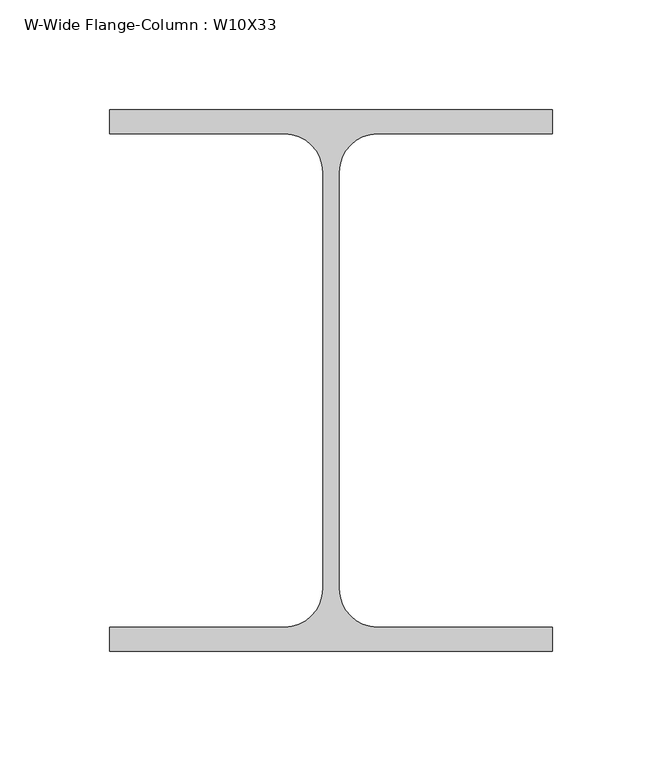
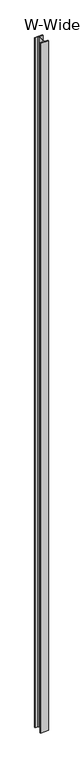
"""IFC4 building model written with IfcOpenShell, lengths in millimetres: column geometry, W-Wide Flange-Column : W10X33."""

from ifc_helpers import new_model, si_unit, point, frame, frame_2d, origin, place, context, project, spatial, polyline, circle_curve, trimmed, segment, composite_curve, outline, extrude, source, transform, mapped, element, save


def w_wide_flange_column_w10x33_d5634f11(model_context):
    return source(origin(), model_context, "Body", "SweptSolid", [
        extrude(outline(composite_curve([segment(polyline([(101.092, 123.571), (101.092, 112.522), (21.209, 112.522)]), True, "CONTINUOUS"), segment(trimmed(circle_curve(frame_2d((21.209, 94.996)), 17.526), [point((21.209, 112.522))], [point((3.683, 94.996))], True, "CARTESIAN"), True, "CONTINUOUS"), segment(polyline([(3.683, 94.996), (3.683, -94.996)]), True, "CONTINUOUS"), segment(trimmed(circle_curve(frame_2d((21.209, -94.996)), 17.526), [point((3.683, -94.996))], [point((21.209, -112.522))], True, "CARTESIAN"), True, "CONTINUOUS"), segment(polyline([(21.209, -112.522), (101.092, -112.522), (101.092, -123.571), (-101.092, -123.571), (-101.092, -112.522), (-21.209, -112.522)]), True, "CONTINUOUS"), segment(trimmed(circle_curve(frame_2d((-21.209, -94.996)), 17.526), [point((-21.209, -112.522))], [point((-3.683, -94.996))], True, "CARTESIAN"), True, "CONTINUOUS"), segment(polyline([(-3.683, -94.996), (-3.683, 94.996)]), True, "CONTINUOUS"), segment(trimmed(circle_curve(frame_2d((-21.209, 94.996)), 17.526), [point((-3.683, 94.996))], [point((-21.209, 112.522))], True, "CARTESIAN"), True, "CONTINUOUS"), segment(polyline([(-21.209, 112.522), (-101.092, 112.522), (-101.092, 123.571), (101.092, 123.571)]), True, "CONTINUOUS")], self_intersect=False)), frame((0.0, 0.0, 9163.05), z_axis=(0.0, 0.0, 1.0), x_axis=(1.0, 0.0, 0.0)), (0.0, 0.0, 1.0), 18421.35),
    ])


if __name__ == "__main__":
    model = new_model("IFC4")
    model_context = context("Model", 3, world=origin())
    ifc_project = project(units=[si_unit("LENGTHUNIT", "METRE", prefix="MILLI")], contexts=[model_context])
    site = spatial("IfcSite", under=ifc_project)
    building = spatial("IfcBuilding", under=site)
    placement = place(None, origin())
    w_wide_flange_column_w10x33_shape = w_wide_flange_column_w10x33_d5634f11(model_context)
    element("IfcColumn", 1, ObjectType="W-Wide Flange-Column : W10X33", at=placement, inside=building, context=model_context, shape_type="MappedRepresentation", body=[
        mapped(w_wide_flange_column_w10x33_shape, transform((0.0, 0.0, 0.0), x_axis=(1.0, 0.0, 0.0), y_axis=(0.0, 1.0, 0.0), z_axis=(0.0, 0.0, 1.0))),
    ])
    save(model, "model.ifc")

# Revit data of these elements
# Type "W-Wide Flange-Column : W10X33"
#   Assembly Code = "B10"
#   W = 33
#   bf = 0' - 7.96"
#   d = 0' - 9.73"
#   k = 0' - 1 1/8"
#   kr = 0' - 0.69"
#   tf = 0' - 0.435"
#   tw = 0' - 0.29"
#   A = 0.0674306 SF
#   Structural Material [instance default] = Steel ASTM A992
# Element 1 (IfcColumn, "W-Wide Flange-Column : W10X33")
#   Materials on its faces: "Steel ASTM A992"
# Materials
#   "Steel ASTM A992": class "Metal", colour RGB 199 199 199, transparency 0, Description = "Structural steel 50ksi", Cost = 0
